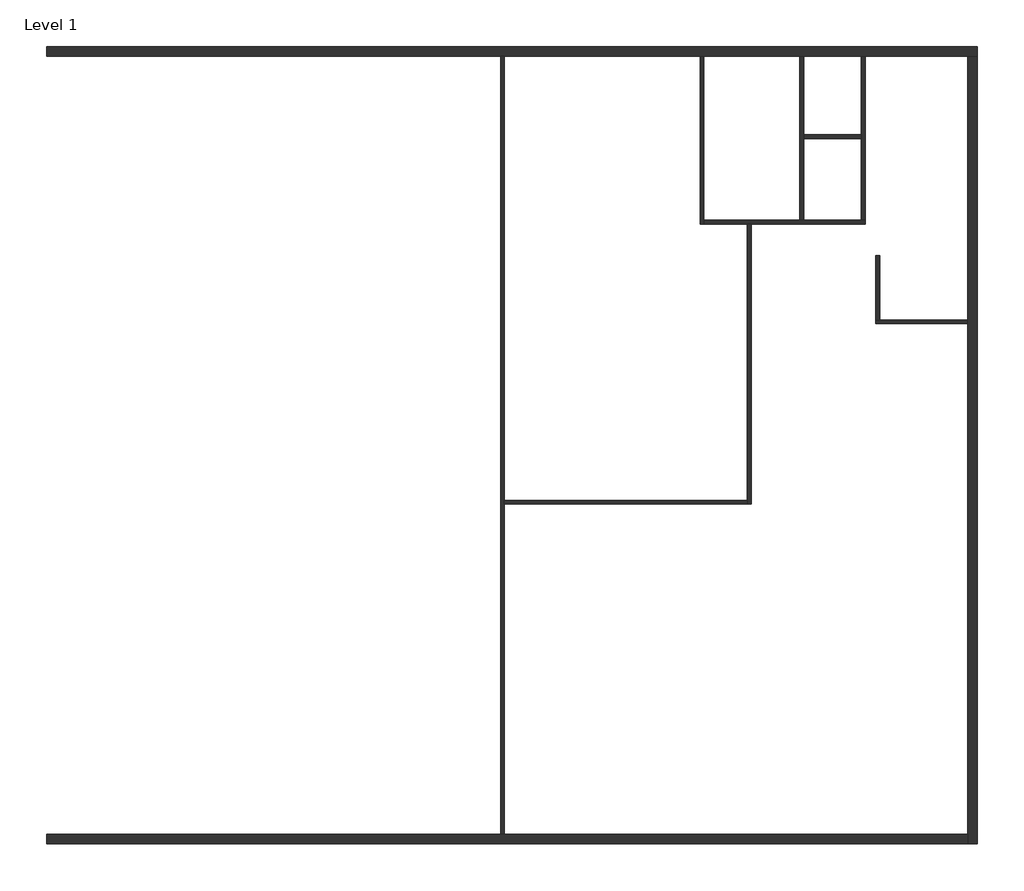
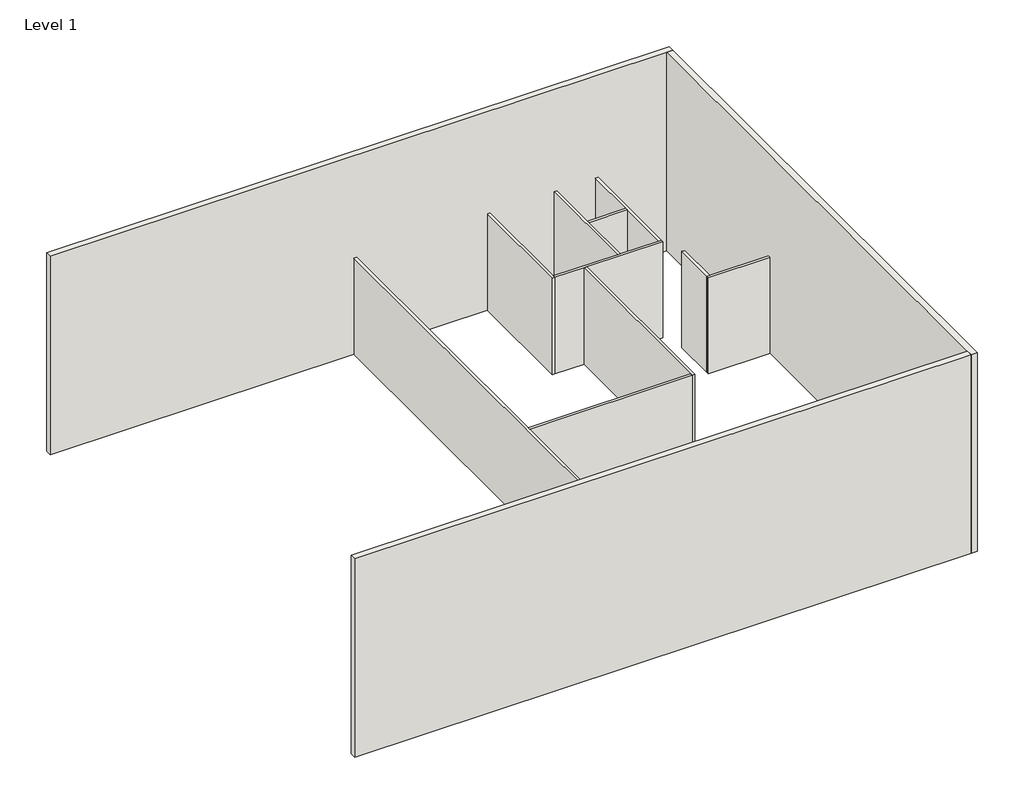
# One storey: 13 walls.
"""IFC4 building model written with IfcOpenShell, lengths in millimetres."""

import ifcopenshell
import ifcopenshell.guid

model = None  # the IFC model being written
_history = None  # IfcOwnerHistory: only IFC2X3 demands one
_inside = {}  # id of a spatial element -> (the spatial element, [elements in it])
_under = {}  # id of a project, library or spatial element -> (it, [spatial elements below it])
_declared = {}  # id of a project -> (the project, [libraries it declares])
_typed = {}  # id of a type object -> (the type object, [elements of that type])
_made_of = {}  # id of a material, layer set ... -> (it, [elements and type objects made of it])


def new_model(schema):
    """Start an empty IFC model of exactly this schema.

    Asked for "IFC4X3", IfcOpenShell would pick the latest addendum, in which some entities
    have other attributes; the version numbers below select the first issue.
    IFC2X3 requires an IfcOwnerHistory on every rooted entity: one is made here for all.
    """
    global model, _history
    if schema == "IFC4X3":
        model = ifcopenshell.file(schema_version=(4, 3, 0, 0))
    else:
        model = ifcopenshell.file(schema=schema)
    _inside.clear()
    _under.clear()
    _declared.clear()
    _typed.clear()
    _made_of.clear()
    _history = None
    if model.schema == "IFC2X3":
        org = make("IfcOrganization", Name="unknown")
        user = make(
            "IfcPersonAndOrganization",
            ThePerson=make("IfcPerson", FamilyName="unknown"),
            TheOrganization=org,
        )
        app = make(
            "IfcApplication",
            ApplicationDeveloper=org,
            Version="unknown",
            ApplicationFullName="unknown",
            ApplicationIdentifier="unknown",
        )
        _history = make(
            "IfcOwnerHistory",
            OwningUser=user,
            OwningApplication=app,
            ChangeAction="ADDED",
            CreationDate=0,
        )
    return model


def make(cls, **values):
    """One entity of the class cls with the attributes given. An attribute that is None is left unset."""
    return model.create_entity(
        cls, **{name: value for name, value in values.items() if value is not None}
    )


def rooted(cls, **values):
    """An entity with a GlobalId (a new one), such as an element, a storey or a relation."""
    return make(cls, GlobalId=ifcopenshell.guid.new(), OwnerHistory=_history, **values)


def si_unit(unit_type, name, prefix=None):
    """IfcSIUnit, for example si_unit("LENGTHUNIT", "METRE", prefix="MILLI")."""
    return make("IfcSIUnit", UnitType=unit_type, Prefix=prefix, Name=name)


def assignment(units):
    """IfcUnitAssignment: the units of a project."""
    return None if units is None else make("IfcUnitAssignment", Units=units)


def point(xyz):
    """IfcCartesianPoint."""
    return None if xyz is None else make("IfcCartesianPoint", Coordinates=xyz)


def direction(xyz):
    """IfcDirection."""
    return None if xyz is None else make("IfcDirection", DirectionRatios=xyz)


def frame(location, z_axis=None, x_axis=None):
    """IfcAxis2Placement3D, a coordinate frame: its origin and axes. An axis left out is left unset."""
    return make(
        "IfcAxis2Placement3D",
        Location=point(location),
        Axis=direction(z_axis),
        RefDirection=direction(x_axis),
    )


def origin():
    """The frame at (0, 0, 0) with its axes left unset."""
    return frame((0.0, 0.0, 0.0))


def origin_with_axes():
    """The frame at (0, 0, 0) with the z axis (0, 0, 1) and the x axis (1, 0, 0) written out."""
    return frame((0.0, 0.0, 0.0), z_axis=(0.0, 0.0, 1.0), x_axis=(1.0, 0.0, 0.0))


def place(relative_to, where):
    """IfcLocalPlacement: puts the frame where relative to a parent placement (None: the world)."""
    return make(
        "IfcLocalPlacement", PlacementRelTo=relative_to, RelativePlacement=where
    )


def context(
    kind, dimensions, precision=None, world=None, true_north=None, identifier=None
):
    """IfcGeometricRepresentationContext, for example the 3D "Model" context."""
    return make(
        "IfcGeometricRepresentationContext",
        ContextIdentifier=identifier,
        ContextType=kind,
        CoordinateSpaceDimension=dimensions,
        Precision=precision,
        WorldCoordinateSystem=world,
        TrueNorth=true_north,
    )


def project(units=None, contexts=None):
    """IfcProject with its units and contexts."""
    return rooted(
        "IfcProject",
        Name="project",
        RepresentationContexts=contexts,
        UnitsInContext=assignment(units),
    )


def spatial(cls, under=None, at=None, **own):
    """A site, building, storey or space (cls), placed at a placement, below another one or the project."""
    s = rooted(cls, ObjectPlacement=at, **own)
    if under is not None:
        _under.setdefault(under.id(), (under, []))[1].append(s)
    return s


def polyline(points):
    """IfcPolyline through the points."""
    return make("IfcPolyline", Points=[point(p) for p in points])


def outline(outer, holes=None, kind="AREA"):
    """IfcArbitraryClosedProfileDef: a profile drawn as a closed curve; with holes, ...WithVoids."""
    if holes is None:
        return make("IfcArbitraryClosedProfileDef", ProfileType=kind, OuterCurve=outer)
    return make(
        "IfcArbitraryProfileDefWithVoids",
        ProfileType=kind,
        OuterCurve=outer,
        InnerCurves=holes,
    )


def extrude(swept, where, along, depth):
    """IfcExtrudedAreaSolid: the profile swept, set in the frame where, extruded along a direction by depth."""
    return make(
        "IfcExtrudedAreaSolid",
        SweptArea=swept,
        Position=where,
        ExtrudedDirection=direction(along),
        Depth=depth,
    )


def faces_of(points, faces, orient=None, outer=None):
    """IfcFace entities. A face is a list of loops; a loop is a list of indices into points, from 0.

    orient and outer hold one flag for each loop. By default every Orientation is true, the
    first loop of a face is its IfcFaceOuterBound and the others are IfcFaceBound.
    """
    made = []
    for i, loops in enumerate(faces):
        bounds = []
        for j, loop in enumerate(loops):
            is_outer = j == 0 if outer is None else outer[i][j]
            bounds.append(
                make(
                    "IfcFaceOuterBound" if is_outer else "IfcFaceBound",
                    Bound=make("IfcPolyLoop", Polygon=[points[k] for k in loop]),
                    Orientation=True if orient is None else orient[i][j],
                )
            )
        made.append(make("IfcFace", Bounds=bounds))
    return made


def faceted_brep(points, faces, orient=None, outer=None, voids=None):
    """IfcFacetedBrep: a solid bounded by flat faces; with voids (closed shells), ...WithVoids."""
    shared = [point(p) for p in points]
    hull = make("IfcClosedShell", CfsFaces=faces_of(shared, faces, orient, outer))
    if voids is None:
        return make("IfcFacetedBrep", Outer=hull)
    return make(
        "IfcFacetedBrepWithVoids",
        Outer=hull,
        Voids=[
            make(cls, CfsFaces=faces_of(shared, fs, o, b)) for cls, fs, o, b in voids
        ],
    )


def shape(context_of_items, identifier, shape_type, items):
    """IfcShapeRepresentation: the items that make up one representation, for example the "Body"."""
    return make(
        "IfcShapeRepresentation",
        ContextOfItems=context_of_items,
        RepresentationIdentifier=identifier,
        RepresentationType=shape_type,
        Items=items,
    )


def made_of(thing, what):
    """Note that an element or type object is made of a material, layer set ...; save() writes the relation."""
    if what is not None:
        _made_of.setdefault(what.id(), (what, []))[1].append(thing)
    return thing


def element(
    cls,
    number,
    at=None,
    inside=None,
    cuts=None,
    type_object=None,
    material=None,
    context=None,
    identifier="Body",
    shape_type=None,
    held_by="IfcProductDefinitionShape",
    body=None,
    shapes=None,
    **own,
):
    """One element of the class cls, such as IfcWall. Its Tag is "e" and its number.

    at: its placement. inside: the storey or other place that contains it. cuts: it is an
    opening in that element (IfcRelVoidsElement). A single representation is given by context,
    identifier, shape_type and body (its items); several are given by shapes. held_by: the class
    of the entity that holds the representations. save() writes the other relations.
    """
    e = rooted(cls, Tag="e%d" % number, ObjectPlacement=at, **own)
    if body is not None:
        shapes = [shape(context, identifier, shape_type, body)]
    if shapes is not None:
        e.Representation = make(held_by, Representations=shapes)
    if inside is not None:
        _inside.setdefault(inside.id(), (inside, []))[1].append(e)
    if cuts is not None:
        rooted(
            "IfcRelVoidsElement", RelatingBuildingElement=cuts, RelatedOpeningElement=e
        )
    if type_object is not None:
        _typed.setdefault(type_object.id(), (type_object, []))[1].append(e)
    return made_of(e, material)


def aggregate(whole, parts):
    """IfcRelAggregates: a whole, such as a stair, and the parts it consists of."""
    return rooted("IfcRelAggregates", RelatingObject=whole, RelatedObjects=parts)


def save(model, path):
    """Write the relations noted so far, then the file.

    IfcRelAggregates (storeys below a building ...), IfcRelContainedInSpatialStructure (elements
    in a storey), IfcRelDefinesByType, IfcRelAssociatesMaterial and IfcRelDeclares: one each for
    every whole, place, type object, material and project.
    """
    for whole, parts in _under.values():
        aggregate(whole, parts)
    for where, things in _inside.values():
        rooted(
            "IfcRelContainedInSpatialStructure",
            RelatedElements=things,
            RelatingStructure=where,
        )
    for kind, things in _typed.values():
        rooted("IfcRelDefinesByType", RelatedObjects=things, RelatingType=kind)
    for what, things in _made_of.values():
        rooted("IfcRelAssociatesMaterial", RelatedObjects=things, RelatingMaterial=what)
    for by, libraries in _declared.values():
        rooted("IfcRelDeclares", RelatingContext=by, RelatedDefinitions=libraries)
    model.write(path)


model = new_model("IFC4")

# Units and contexts
model_context = context("Model", 3, world=origin())
ifc_project = project(units=[si_unit("LENGTHUNIT", "METRE", prefix="MILLI")], contexts=[model_context])

# Site, building, storey
site = spatial("IfcSite", under=ifc_project)
building = spatial("IfcBuilding", under=site)
storey = spatial("IfcBuildingStorey", under=building, Name="Level 1", Elevation=0.0)

# Walls
placement = place(None, origin())
element("IfcWall", 1, ObjectType="Generic - 12\"", at=placement, inside=storey, context=model_context, shape_type="Brep", body=[
    faceted_brep([(-11486.7262822, 13482.5120281, 0.0), (3080.1737178, 13482.5120281, 0.0), (3207.1737178, 13482.5120281, 0.0), (9480.9737178, 13482.5120281, 0.0), (9607.9737178, 13482.5120281, 0.0), (12681.3737178, 13482.5120281, 0.0), (12808.3737178, 13482.5120281, 0.0), (14662.5737178, 13482.5120281, 0.0), (14789.5737178, 13482.5120281, 0.0), (18078.8737178, 13482.5120281, 0.0), (18383.6737178, 13482.5120281, 0.0), (18383.6737178, 13482.5120281, 10058.4), (18078.8737178, 13482.5120281, 10058.4), (-11486.7262822, 13482.5120281, 10058.4), (-11486.7262822, 13787.3120281, 0.0), (-11486.7262822, 13787.3120281, 10058.4), (18383.6737178, 13787.3120281, 10058.4), (18383.6737178, 13787.3120281, 0.0)], [[[0, 1, 2, 3, 4, 5, 6, 7, 8, 9, 10, 11, 12, 13]], [[14, 15, 16, 17]], [[10, 9, 8, 7, 6, 5, 4, 3, 2, 1, 0, 14, 17]], [[13, 12, 11, 16, 15]], [[0, 13, 15, 14]], [[11, 10, 17, 16]]]),
])
element("IfcWall", 2, ObjectType="Generic - 12\"", at=placement, inside=storey, context=model_context, shape_type="Brep", body=[
    faceted_brep([(18078.8737178, 13482.5120281, 0.0), (18078.8737178, 5011.6120281, 0.0), (18078.8737178, 4884.6120281, 0.0), (18078.8737178, -11511.0879719, 0.0), (18078.8737178, -11815.8879719, 0.0), (18078.8737178, -11815.8879719, 10058.4), (18078.8737178, -11511.0879719, 10058.4), (18078.8737178, 13482.5120281, 10058.4), (18383.6737178, 13482.5120281, 0.0), (18383.6737178, 13482.5120281, 10058.4), (18383.6737178, -11815.8879719, 10058.4), (18383.6737178, -11815.8879719, 0.0)], [[[0, 1, 2, 3, 4, 5, 6, 7]], [[8, 9, 10, 11]], [[4, 3, 2, 1, 0, 8, 11]], [[7, 6, 5, 10, 9]], [[0, 7, 9, 8]], [[5, 4, 11, 10]]]),
])
element("IfcWall", 3, ObjectType="Generic - 12\"", at=placement, inside=storey, context=model_context, shape_type="Brep", body=[
    faceted_brep([(18078.8737178, -11511.0879719, 0.0), (3207.1737178, -11511.0879719, 0.0), (3080.1737178, -11511.0879719, 0.0), (-11486.7262822, -11511.0879719, 0.0), (-11486.7262822, -11511.0879719, 10058.4), (18078.8737178, -11511.0879719, 10058.4), (18078.8737178, -11815.8879719, 0.0), (18078.8737178, -11815.8879719, 10058.4), (-11486.7262822, -11815.8879719, 10058.4), (-11486.7262822, -11815.8879719, 0.0)], [[[0, 1, 2, 3, 4, 5]], [[6, 7, 8, 9]], [[3, 2, 1, 0, 6, 9]], [[4, 3, 9, 8]], [[5, 4, 8, 7]], [[0, 5, 7, 6]]]),
])
element("IfcWall", 4, ObjectType="Generic - 5\"", at=placement, inside=storey, context=model_context, shape_type="Brep", body=[
    faceted_brep([(3207.1737178, -11511.0879719, 0.0), (3207.1737178, -906.5879719, 0.0), (3207.1737178, -779.5879719, 0.0), (3207.1737178, 13482.5120281, 0.0), (3207.1737178, 13482.5120281, 4876.8), (3207.1737178, -779.5879719, 4876.8), (3207.1737178, -906.5879719, 4876.8), (3207.1737178, -11511.0879719, 4876.8), (3080.1737178, -11511.0879719, 0.0), (3080.1737178, -11511.0879719, 4876.8), (3080.1737178, 13482.5120281, 4876.8), (3080.1737178, 13482.5120281, 0.0)], [[[0, 1, 2, 3, 4, 5, 6, 7]], [[8, 9, 10, 11]], [[3, 2, 1, 0, 8, 11]], [[7, 6, 5, 4, 10, 9]], [[4, 3, 11, 10]], [[0, 7, 9, 8]]]),
])
element("IfcWall", 5, ObjectType="Generic - 5\"", at=placement, inside=storey, context=model_context, shape_type="Brep", body=[
    faceted_brep([(9480.9737178, 13482.5120281, 0.0), (9480.9737178, 8085.0120281, 0.0), (9480.9737178, 8085.0120281, 4876.8), (9480.9737178, 13482.5120281, 4876.8), (9607.9737178, 13482.5120281, 0.0), (9607.9737178, 13482.5120281, 4876.8), (9607.9737178, 8212.0120281, 4876.8), (9607.9737178, 8085.0120281, 4876.8), (9607.9737178, 8085.0120281, 0.0), (9607.9737178, 8212.0120281, 0.0)], [[[0, 1, 2, 3]], [[4, 5, 6, 7, 8, 9]], [[1, 0, 4, 9, 8]], [[3, 2, 7, 6, 5]], [[0, 3, 5, 4]], [[2, 1, 8, 7]]]),
])
element("IfcWall", 6, ObjectType="Generic - 5\"", at=placement, inside=storey, context=model_context, shape_type="Brep", body=[
    faceted_brep([(9607.9737178, 8085.0120281, 0.0), (11004.9737178, 8085.0120281, 0.0), (11131.9737178, 8085.0120281, 0.0), (14789.5737178, 8085.0120281, 0.0), (14789.5737178, 8085.0120281, 4876.8), (11131.9737178, 8085.0120281, 4876.8), (11004.9737178, 8085.0120281, 4876.8), (9607.9737178, 8085.0120281, 4876.8), (9607.9737178, 8212.0120281, 0.0), (9607.9737178, 8212.0120281, 4876.8), (12681.3737178, 8212.0120281, 4876.8), (12808.3737178, 8212.0120281, 4876.8), (14662.5737178, 8212.0120281, 4876.8), (14789.5737178, 8212.0120281, 4876.8), (14789.5737178, 8212.0120281, 0.0), (14662.5737178, 8212.0120281, 0.0), (12808.3737178, 8212.0120281, 0.0), (12681.3737178, 8212.0120281, 0.0)], [[[0, 1, 2, 3, 4, 5, 6, 7]], [[8, 9, 10, 11, 12, 13, 14, 15, 16, 17]], [[3, 2, 1, 0, 8, 17, 16, 15, 14]], [[7, 6, 5, 4, 13, 12, 11, 10, 9]], [[0, 7, 9, 8]], [[4, 3, 14, 13]]]),
])
element("IfcWall", 7, ObjectType="Generic - 5\"", at=placement, inside=storey, context=model_context, shape_type="Brep", body=[
    faceted_brep([(14789.5737178, 8212.0120281, 0.0), (14789.5737178, 13482.5120281, 0.0), (14789.5737178, 13482.5120281, 4876.8), (14789.5737178, 8212.0120281, 4876.8), (14662.5737178, 8212.0120281, 0.0), (14662.5737178, 8212.0120281, 4876.8), (14662.5737178, 10828.2120281, 4876.8), (14662.5737178, 10955.2120281, 4876.8), (14662.5737178, 13482.5120281, 4876.8), (14662.5737178, 13482.5120281, 0.0), (14662.5737178, 10955.2120281, 0.0), (14662.5737178, 10828.2120281, 0.0)], [[[0, 1, 2, 3]], [[4, 5, 6, 7, 8, 9, 10, 11]], [[1, 0, 4, 11, 10, 9]], [[3, 2, 8, 7, 6, 5]], [[0, 3, 5, 4]], [[2, 1, 9, 8]]]),
])
element("IfcWall", 8, ObjectType="Generic - 5\"", at=placement, inside=storey, context=model_context, shape_type="Brep", body=[
    faceted_brep([(12681.3737178, 13482.5120281, 0.0), (12681.3737178, 8212.0120281, 0.0), (12681.3737178, 8212.0120281, 4876.8), (12681.3737178, 13482.5120281, 4876.8), (12808.3737178, 13482.5120281, 0.0), (12808.3737178, 13482.5120281, 4876.8), (12808.3737178, 10955.2120281, 4876.8), (12808.3737178, 10828.2120281, 4876.8), (12808.3737178, 8212.0120281, 4876.8), (12808.3737178, 8212.0120281, 0.0), (12808.3737178, 10828.2120281, 0.0), (12808.3737178, 10955.2120281, 0.0)], [[[0, 1, 2, 3]], [[4, 5, 6, 7, 8, 9, 10, 11]], [[1, 0, 4, 11, 10, 9]], [[3, 2, 8, 7, 6, 5]], [[0, 3, 5, 4]], [[2, 1, 9, 8]]]),
])
element("IfcWall", 9, ObjectType="Generic - 5\"", at=placement, inside=storey, context=model_context, shape_type="SweptSolid", body=[
    extrude(outline(polyline([(12808.3737178, 10955.2120281), (14662.5737178, 10955.2120281), (14662.5737178, 10828.2120281), (12808.3737178, 10828.2120281), (12808.3737178, 10955.2120281)])), origin_with_axes(), (0.0, 0.0, 1.0), 4876.8),
])
element("IfcWall", 10, ObjectType="Generic - 5\"", at=placement, inside=storey, context=model_context, shape_type="Brep", body=[
    faceted_brep([(18078.8737178, 5011.6120281, 0.0), (15246.7737178, 5011.6120281, 0.0), (15119.7737178, 5011.6120281, 0.0), (15119.7737178, 5011.6120281, 4876.8), (15246.7737178, 5011.6120281, 4876.8), (18078.8737178, 5011.6120281, 4876.8), (18078.8737178, 4884.6120281, 0.0), (18078.8737178, 4884.6120281, 4876.8), (15119.7737178, 4884.6120281, 4876.8), (15119.7737178, 4884.6120281, 0.0)], [[[0, 1, 2, 3, 4, 5]], [[6, 7, 8, 9]], [[2, 1, 0, 6, 9]], [[5, 4, 3, 8, 7]], [[0, 5, 7, 6]], [[3, 2, 9, 8]]]),
])
element("IfcWall", 11, ObjectType="Generic - 5\"", at=placement, inside=storey, context=model_context, shape_type="SweptSolid", body=[
    extrude(outline(polyline([(15246.7737178, 7081.7120281), (15246.7737178, 5011.6120281), (15119.7737178, 5011.6120281), (15119.7737178, 7081.7120281), (15246.7737178, 7081.7120281)])), origin_with_axes(), (0.0, 0.0, 1.0), 4876.8),
])
element("IfcWall", 12, ObjectType="Generic - 5\"", at=placement, inside=storey, context=model_context, shape_type="Brep", body=[
    faceted_brep([(11004.9737178, 8085.0120281, 0.0), (11004.9737178, -779.5879719, 0.0), (11004.9737178, -906.5879719, 0.0), (11004.9737178, -906.5879719, 4876.8), (11004.9737178, -779.5879719, 4876.8), (11004.9737178, 8085.0120281, 4876.8), (11131.9737178, 8085.0120281, 0.0), (11131.9737178, 8085.0120281, 4876.8), (11131.9737178, -906.5879719, 4876.8), (11131.9737178, -906.5879719, 0.0)], [[[0, 1, 2, 3, 4, 5]], [[6, 7, 8, 9]], [[2, 1, 0, 6, 9]], [[5, 4, 3, 8, 7]], [[0, 5, 7, 6]], [[3, 2, 9, 8]]]),
])
element("IfcWall", 13, ObjectType="Generic - 5\"", at=placement, inside=storey, context=model_context, shape_type="SweptSolid", body=[
    extrude(outline(polyline([(3207.1737178, -779.5879719), (11004.9737178, -779.5879719), (11004.9737178, -906.5879719), (3207.1737178, -906.5879719), (3207.1737178, -779.5879719)])), origin_with_axes(), (0.0, 0.0, 1.0), 4876.8),
])

save(model, "model.ifc")

# Revit data of these elements
# Project information
#   Project Issue Date = "Issue Date"
#   Project Status = "Project Status"
#   Client Name = "Owner"
#   Project Address = "Enter address here"
#   Project Name = "Project Name"
#   Project Number = "Project Number"
# Grids (mm)
#   "1": line (-18801.926, 15817.913) -> (-18801.926, -14896.109)
#   "2": line (-11486.726, 15817.913) -> (-11486.726, -14896.109)
#   "3": line (-4171.526, 15817.913) -> (-4171.526, -14896.109)
#   "4": line (3143.674, 15817.913) -> (3143.674, -14896.109)
#   "5": line (10458.874, 15817.913) -> (10458.874, -14896.109)
#   "6": line (17774.074, 15817.913) -> (17774.074, -14896.109)
#   "A": line (23913.763, 13177.712) -> (-22245.007, 13177.712)
#   "B": line (23913.763, 5862.512) -> (-22245.007, 5862.512)
#   "C": line (23913.763, -2671.888) -> (-22245.007, -2671.888)
#   "D": line (23913.763, -11206.288) -> (-22245.007, -11206.288)
# Type "Generic - 12\""
#   Assembly Code = "B2010"
#   Layers, outside or top first: 1' - 0" no material (function 1)
# Type "Generic - 5\""
#   Assembly Code = "B2010"
#   Layers, outside or top first: 0' - 5" no material (function 1)
# Elements 1, 2, 3 (IfcWall, "Generic - 12\"")
#   Top Offset = 0' - 0"
#   Base Offset = 0' - 0"
#   wall height = 33' - 0"
#   Phase Created = New Construction
#   Base Constraint = Level 1
#   Top Constraint = Parapet
#   Materials on its faces: "Default Wall"
# Elements 4, 5, 6, 7, 8, 9, 10, 11, 12, 13 (IfcWall, "Generic - 5\"")
#   Top Offset = 0' - 0"
#   Base Offset = 0' - 0"
#   wall height = 16' - 0"
#   Phase Created = New Construction
#   Base Constraint = Level 1
#   Top Constraint = Level 2
#   Materials on its faces: "Default Wall"
# Materials
#   "Default Wall": class "Miscellaneous", colour RGB 127 127 127, transparency 0, Cost = 0
